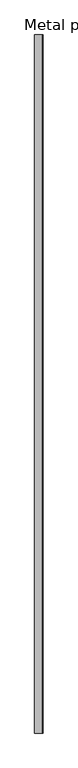
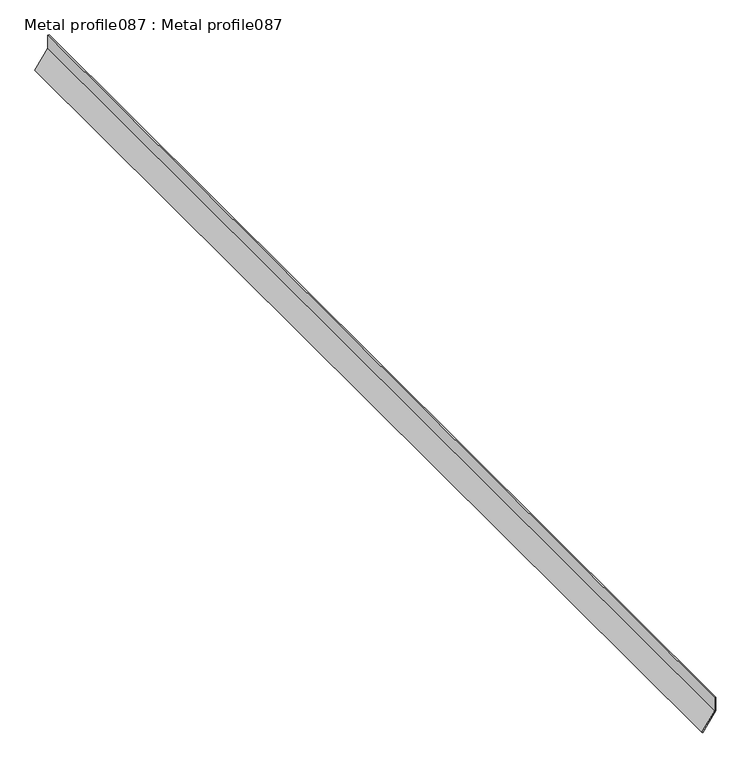
"""IFC4 building model written with IfcOpenShell, lengths in millimetres: proxy geometry, Metal profile087 : Metal profile087."""

from ifc_helpers import new_model, si_unit, frame, origin, place, context, project, spatial, polyline, outline, extrude, source, transform, mapped, element, save


def metal_profile087_metal_profile087_4ebeef7e(model_context):
    return source(origin(), model_context, "Body", "SweptSolid", [
        extrude(outline(polyline([(42168.484375, -2462.7717285), (42144.6612907, -2462.7717285), (42112.5174165, -2485.2548518), (42111.3710937, -2483.6159668), (42144.03125, -2460.7717285), (42168.484375, -2460.7717285), (42168.484375, -2462.7717285)])), frame((0.0, -1052.8906574, 0.0), z_axis=(0.0, 1.0, 0.0), x_axis=(0.0, 0.0, 1.0)), (0.0, 0.0, 1.0), 2000.0),
    ])


if __name__ == "__main__":
    model = new_model("IFC4")
    model_context = context("Model", 3, world=origin())
    ifc_project = project(units=[si_unit("LENGTHUNIT", "METRE", prefix="MILLI")], contexts=[model_context])
    site = spatial("IfcSite", under=ifc_project)
    building = spatial("IfcBuilding", under=site)
    placement = place(None, origin())
    metal_profile087_metal_profile087_shape = metal_profile087_metal_profile087_4ebeef7e(model_context)
    element("IfcBuildingElementProxy", 1, Name="Metal profile087 : Metal profile087", ObjectType="Metal profile087 : Metal profile087", at=placement, inside=building, context=model_context, shape_type="MappedRepresentation", body=[
        mapped(metal_profile087_metal_profile087_shape, transform((0.0, 0.0, 0.0), x_axis=(1.0, 0.0, 0.0), y_axis=(0.0, 1.0, 0.0), z_axis=(0.0, 0.0, 1.0))),
    ])
    save(model, "model.ifc")

# Revit data of these elements
# Type "Metal profile087 : Metal profile087"
#   NameOverride = "Metal profile087"
# Element 1 (IfcBuildingElementProxy, "Metal profile087 : Metal profile087")
#   Materials on its faces: "TRIM CLEAT"
# Materials
#   "TRIM CLEAT": class "Unassigned", colour RGB 255 232 5, transparency 0
